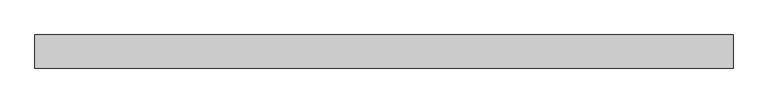
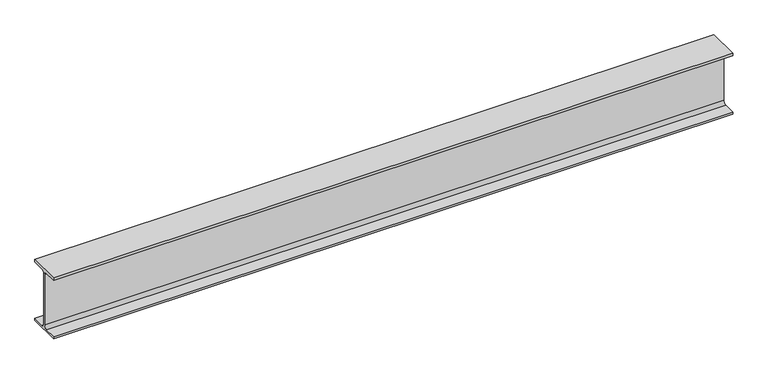
"""IFC4 building model written with IfcOpenShell, lengths in millimetres: beam geometry, 0912_Steel Framing_H-KSD3502 : H_SB_ASB_H-250x125x6x9."""

import ifcopenshell
import ifcopenshell.guid

model = None  # the IFC model being written
_history = None  # IfcOwnerHistory: only IFC2X3 demands one
_inside = {}  # id of a spatial element -> (the spatial element, [elements in it])
_under = {}  # id of a project, library or spatial element -> (it, [spatial elements below it])
_declared = {}  # id of a project -> (the project, [libraries it declares])
_typed = {}  # id of a type object -> (the type object, [elements of that type])
_made_of = {}  # id of a material, layer set ... -> (it, [elements and type objects made of it])


def new_model(schema):
    """Start an empty IFC model of exactly this schema.

    Asked for "IFC4X3", IfcOpenShell would pick the latest addendum, in which some entities
    have other attributes; the version numbers below select the first issue.
    IFC2X3 requires an IfcOwnerHistory on every rooted entity: one is made here for all.
    """
    global model, _history
    if schema == "IFC4X3":
        model = ifcopenshell.file(schema_version=(4, 3, 0, 0))
    else:
        model = ifcopenshell.file(schema=schema)
    _inside.clear()
    _under.clear()
    _declared.clear()
    _typed.clear()
    _made_of.clear()
    _history = None
    if model.schema == "IFC2X3":
        org = make("IfcOrganization", Name="unknown")
        user = make(
            "IfcPersonAndOrganization",
            ThePerson=make("IfcPerson", FamilyName="unknown"),
            TheOrganization=org,
        )
        app = make(
            "IfcApplication",
            ApplicationDeveloper=org,
            Version="unknown",
            ApplicationFullName="unknown",
            ApplicationIdentifier="unknown",
        )
        _history = make(
            "IfcOwnerHistory",
            OwningUser=user,
            OwningApplication=app,
            ChangeAction="ADDED",
            CreationDate=0,
        )
    return model


def make(cls, **values):
    """One entity of the class cls with the attributes given. An attribute that is None is left unset."""
    return model.create_entity(
        cls, **{name: value for name, value in values.items() if value is not None}
    )


def rooted(cls, **values):
    """An entity with a GlobalId (a new one), such as an element, a storey or a relation."""
    return make(cls, GlobalId=ifcopenshell.guid.new(), OwnerHistory=_history, **values)


def si_unit(unit_type, name, prefix=None):
    """IfcSIUnit, for example si_unit("LENGTHUNIT", "METRE", prefix="MILLI")."""
    return make("IfcSIUnit", UnitType=unit_type, Prefix=prefix, Name=name)


def assignment(units):
    """IfcUnitAssignment: the units of a project."""
    return None if units is None else make("IfcUnitAssignment", Units=units)


def point(xyz):
    """IfcCartesianPoint."""
    return None if xyz is None else make("IfcCartesianPoint", Coordinates=xyz)


def direction(xyz):
    """IfcDirection."""
    return None if xyz is None else make("IfcDirection", DirectionRatios=xyz)


def frame(location, z_axis=None, x_axis=None):
    """IfcAxis2Placement3D, a coordinate frame: its origin and axes. An axis left out is left unset."""
    return make(
        "IfcAxis2Placement3D",
        Location=point(location),
        Axis=direction(z_axis),
        RefDirection=direction(x_axis),
    )


def frame_2d(location, x_axis=None):
    """IfcAxis2Placement2D, a coordinate frame in the plane: its origin and x axis."""
    return make(
        "IfcAxis2Placement2D", Location=point(location), RefDirection=direction(x_axis)
    )


def origin():
    """The frame at (0, 0, 0) with its axes left unset."""
    return frame((0.0, 0.0, 0.0))


def place(relative_to, where):
    """IfcLocalPlacement: puts the frame where relative to a parent placement (None: the world)."""
    return make(
        "IfcLocalPlacement", PlacementRelTo=relative_to, RelativePlacement=where
    )


def context(
    kind, dimensions, precision=None, world=None, true_north=None, identifier=None
):
    """IfcGeometricRepresentationContext, for example the 3D "Model" context."""
    return make(
        "IfcGeometricRepresentationContext",
        ContextIdentifier=identifier,
        ContextType=kind,
        CoordinateSpaceDimension=dimensions,
        Precision=precision,
        WorldCoordinateSystem=world,
        TrueNorth=true_north,
    )


def project(units=None, contexts=None):
    """IfcProject with its units and contexts."""
    return rooted(
        "IfcProject",
        Name="project",
        RepresentationContexts=contexts,
        UnitsInContext=assignment(units),
    )


def spatial(cls, under=None, at=None, **own):
    """A site, building, storey or space (cls), placed at a placement, below another one or the project."""
    s = rooted(cls, ObjectPlacement=at, **own)
    if under is not None:
        _under.setdefault(under.id(), (under, []))[1].append(s)
    return s


def polyline(points):
    """IfcPolyline through the points."""
    return make("IfcPolyline", Points=[point(p) for p in points])


def circle_curve(where, radius):
    """IfcCircle in the frame where."""
    return make("IfcCircle", Position=where, Radius=radius)


def trimmed(basis, trim1, trim2, sense, master):
    """IfcTrimmedCurve: the piece of a basis curve between two trims."""
    return make(
        "IfcTrimmedCurve",
        BasisCurve=basis,
        Trim1=trim1,
        Trim2=trim2,
        SenseAgreement=sense,
        MasterRepresentation=master,
    )


def segment(curve, same_sense, transition):
    """IfcCompositeCurveSegment."""
    return make(
        "IfcCompositeCurveSegment",
        Transition=transition,
        SameSense=same_sense,
        ParentCurve=curve,
    )


def composite_curve(segments, self_intersect=None):
    """IfcCompositeCurve: segments joined end to end."""
    return make("IfcCompositeCurve", Segments=segments, SelfIntersect=self_intersect)


def outline(outer, holes=None, kind="AREA"):
    """IfcArbitraryClosedProfileDef: a profile drawn as a closed curve; with holes, ...WithVoids."""
    if holes is None:
        return make("IfcArbitraryClosedProfileDef", ProfileType=kind, OuterCurve=outer)
    return make(
        "IfcArbitraryProfileDefWithVoids",
        ProfileType=kind,
        OuterCurve=outer,
        InnerCurves=holes,
    )


def extrude(swept, where, along, depth):
    """IfcExtrudedAreaSolid: the profile swept, set in the frame where, extruded along a direction by depth."""
    return make(
        "IfcExtrudedAreaSolid",
        SweptArea=swept,
        Position=where,
        ExtrudedDirection=direction(along),
        Depth=depth,
    )


def shape(context_of_items, identifier, shape_type, items):
    """IfcShapeRepresentation: the items that make up one representation, for example the "Body"."""
    return make(
        "IfcShapeRepresentation",
        ContextOfItems=context_of_items,
        RepresentationIdentifier=identifier,
        RepresentationType=shape_type,
        Items=items,
    )


def source(mapping_origin, context_of_items, identifier, shape_type, items):
    """IfcRepresentationMap: a shape defined once, which mapped items show again and again."""
    return make(
        "IfcRepresentationMap",
        MappingOrigin=mapping_origin,
        MappedRepresentation=shape(context_of_items, identifier, shape_type, items),
    )


def transform(
    local_origin,
    x_axis=None,
    y_axis=None,
    z_axis=None,
    scale=None,
    scale2=None,
    scale3=None,
    uniform=True,
):
    """IfcCartesianTransformationOperator3D, or its non-uniform kind. x_axis, y_axis, z_axis: its Axis1, 2, 3."""
    if uniform:
        return make(
            "IfcCartesianTransformationOperator3D",
            Axis1=direction(x_axis),
            Axis2=direction(y_axis),
            LocalOrigin=point(local_origin),
            Scale=scale,
            Axis3=direction(z_axis),
        )
    return make(
        "IfcCartesianTransformationOperator3DnonUniform",
        Axis1=direction(x_axis),
        Axis2=direction(y_axis),
        LocalOrigin=point(local_origin),
        Scale=scale,
        Axis3=direction(z_axis),
        Scale2=scale2,
        Scale3=scale3,
    )


def mapped(mapping_source, mapping_target):
    """IfcMappedItem: shows the shape of a source again, moved by a transform."""
    return make(
        "IfcMappedItem", MappingSource=mapping_source, MappingTarget=mapping_target
    )


def made_of(thing, what):
    """Note that an element or type object is made of a material, layer set ...; save() writes the relation."""
    if what is not None:
        _made_of.setdefault(what.id(), (what, []))[1].append(thing)
    return thing


def element(
    cls,
    number,
    at=None,
    inside=None,
    cuts=None,
    type_object=None,
    material=None,
    context=None,
    identifier="Body",
    shape_type=None,
    held_by="IfcProductDefinitionShape",
    body=None,
    shapes=None,
    **own,
):
    """One element of the class cls, such as IfcWall. Its Tag is "e" and its number.

    at: its placement. inside: the storey or other place that contains it. cuts: it is an
    opening in that element (IfcRelVoidsElement). A single representation is given by context,
    identifier, shape_type and body (its items); several are given by shapes. held_by: the class
    of the entity that holds the representations. save() writes the other relations.
    """
    e = rooted(cls, Tag="e%d" % number, ObjectPlacement=at, **own)
    if body is not None:
        shapes = [shape(context, identifier, shape_type, body)]
    if shapes is not None:
        e.Representation = make(held_by, Representations=shapes)
    if inside is not None:
        _inside.setdefault(inside.id(), (inside, []))[1].append(e)
    if cuts is not None:
        rooted(
            "IfcRelVoidsElement", RelatingBuildingElement=cuts, RelatedOpeningElement=e
        )
    if type_object is not None:
        _typed.setdefault(type_object.id(), (type_object, []))[1].append(e)
    return made_of(e, material)


def aggregate(whole, parts):
    """IfcRelAggregates: a whole, such as a stair, and the parts it consists of."""
    return rooted("IfcRelAggregates", RelatingObject=whole, RelatedObjects=parts)


def save(model, path):
    """Write the relations noted so far, then the file.

    IfcRelAggregates (storeys below a building ...), IfcRelContainedInSpatialStructure (elements
    in a storey), IfcRelDefinesByType, IfcRelAssociatesMaterial and IfcRelDeclares: one each for
    every whole, place, type object, material and project.
    """
    for whole, parts in _under.values():
        aggregate(whole, parts)
    for where, things in _inside.values():
        rooted(
            "IfcRelContainedInSpatialStructure",
            RelatedElements=things,
            RelatingStructure=where,
        )
    for kind, things in _typed.values():
        rooted("IfcRelDefinesByType", RelatedObjects=things, RelatingType=kind)
    for what, things in _made_of.values():
        rooted("IfcRelAssociatesMaterial", RelatedObjects=things, RelatingMaterial=what)
    for by, libraries in _declared.values():
        rooted("IfcRelDeclares", RelatingContext=by, RelatedDefinitions=libraries)
    model.write(path)


def beam_dbfcdd3c(model_context):
    return source(origin(), model_context, "Body", "SweptSolid", [
        extrude(outline(composite_curve([segment(polyline([(62.5, -116.0), (62.5, -125.0), (-62.5, -125.0), (-62.5, -116.0), (-15.0, -116.0)]), True, "CONTINUOUS"), segment(trimmed(circle_curve(frame_2d((-15.0, -104.0)), 12.0), [point((-15.0, -116.0))], [point((-3.0, -104.0))], True, "CARTESIAN"), True, "CONTINUOUS"), segment(polyline([(-3.0, -104.0), (-3.0, 104.0)]), True, "CONTINUOUS"), segment(trimmed(circle_curve(frame_2d((-15.0, 104.0)), 12.0), [point((-3.0, 104.0))], [point((-15.0, 116.0))], True, "CARTESIAN"), True, "CONTINUOUS"), segment(polyline([(-15.0, 116.0), (-62.5, 116.0), (-62.5, 125.0), (62.5, 125.0), (62.5, 116.0), (15.0, 116.0)]), True, "CONTINUOUS"), segment(trimmed(circle_curve(frame_2d((15.0, 104.0)), 12.0), [point((15.0, 116.0))], [point((3.0, 104.0))], True, "CARTESIAN"), True, "CONTINUOUS"), segment(polyline([(3.0, 104.0), (3.0, -104.0)]), True, "CONTINUOUS"), segment(trimmed(circle_curve(frame_2d((15.0, -104.0)), 12.0), [point((3.0, -104.0))], [point((15.0, -116.0))], True, "CARTESIAN"), True, "CONTINUOUS"), segment(polyline([(15.0, -116.0), (62.5, -116.0)]), True, "CONTINUOUS")], self_intersect=False)), frame((-1249.3, 0.0, 0.0), z_axis=(1.0, 0.0, 0.0), x_axis=(0.0, 1.0, 0.0)), (0.0, 0.0, 1.0), 2636.6),
    ])


if __name__ == "__main__":
    model = new_model("IFC4")
    model_context = context("Model", 3, world=origin())
    ifc_project = project(units=[si_unit("LENGTHUNIT", "METRE", prefix="MILLI")], contexts=[model_context])
    site = spatial("IfcSite", under=ifc_project)
    building = spatial("IfcBuilding", under=site)
    placement = place(None, origin())
    beam_shape = beam_dbfcdd3c(model_context)
    element("IfcBeam", 1, ObjectType="0912_Steel Framing_H-KSD3502 : H_SB_ASB_H-250x125x6x9", at=placement, inside=building, context=model_context, shape_type="MappedRepresentation", body=[
        mapped(beam_shape, transform((0.0, 0.0, 0.0), x_axis=(1.0, 0.0, 0.0), y_axis=(0.0, 1.0, 0.0), z_axis=(0.0, 0.0, 1.0))),
    ])
    save(model, "model.ifc")

# Revit data of these elements
# Type "0912_Steel Framing_H-KSD3502 : H_SB_ASB_H-250x125x6x9"
#   H_WM Code_1 = "S01AA003-00001 | Main Steel Structure Fabrication Work | Shelter/Building | Light Steel - Standard (30KG/M>Weight) | Material: (   )"
#   H_WM Code_2 = "S03AA029-00001 | Main Steel Structure Erection Work | Shelter/Building | Light Steel (30KG/M>Weight) | Material: (   )"
#   H_WM Code_3 = "S01AA010-00001 | Main Steel Structure Fabrication Work | Shelter/Building | Steel Painting/Coating | for Non-Fireproofed Steel Surface, Surface Preparation, Primer, Second & Final Coat | Material: (   )"
#   H_Q'ty Cal Type Tag = "SB-Q2"
#   Width = 12.5 cm
#   Web Thickness = 0.6 cm
#   Web Fillet = 1.2 cm
#   Warping Constant = 42539.8 cm⁶
#   W = 0
#   Torsional Moment of Inertia = 7.8102 cm⁴
#   Section Area = 37.66 cm²
#   Plastic Modulus weak axis = 73.1 cm³
#   Plastic Modulus strong axis = 366.0 cm³
#   Perimeter = 0.97 m²/m
#   Nominal Weight = 29.60 kgf/m
#   Moment of Inertia weak axis = 294.00 cm⁴
#   Moment of Inertia strong axis = 4050.00 cm⁴
#   Height = 25.0 cm
#   Flange Thickness = 0.9 cm
#   Elastic Modulus weak axis = 47.0 cm³
#   Elastic Modulus strong axis = 324.0 cm³
#   Centroid Vertical = 12.5 cm
#   Centroid Horizontal = 6.25 cm
#   Ix = 40500000
#   Length [instance default] = 1.5240 m
#   Zx = 366000
#   b = 0.1250 m
#   h = 0.2500 m
#   r = 0.0120 m
#   s = 0.0060 m
#   t = 0.0090 m
#   A = 0.003766 m²
#   Structural Material [instance default] = Steel, 45-345
#   Assembly Code = ""
# Element 1 (IfcBeam, "0912_Steel Framing_H-KSD3502 : H_SB_ASB_H-250x125x6x9")
#   Structural Material = none
# Materials
#   "Steel, 45-345": class "Metal", colour RGB 189 187 185, transparency 0, Description = "Steel 345 MPa", Cost = 0
